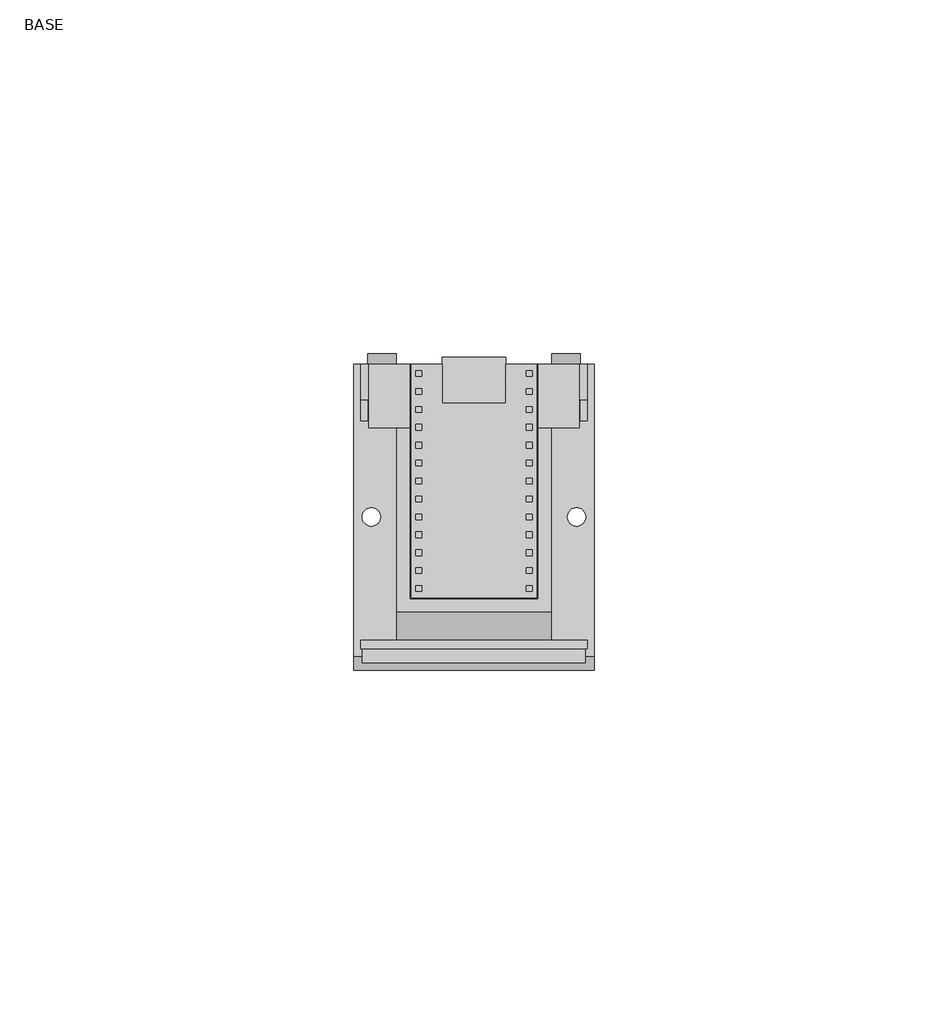
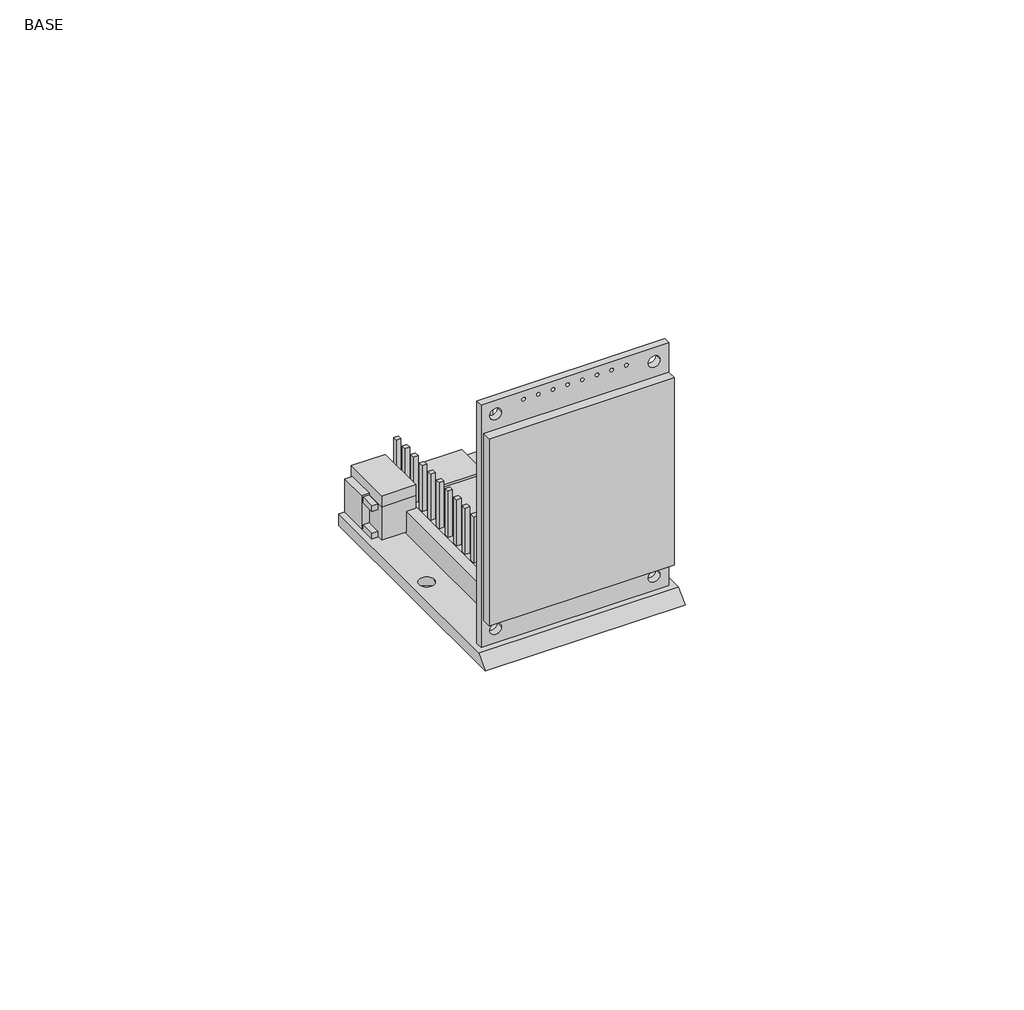
# One storey: 4 furniture elements, 1 proxy.
# Revit data of these elements (continued)
# Element 2 (IfcFurniture, "1.54TFT_SCREEN : 1.54TFT_SCREEN")
#   Phase Created = Fase 1
#   Materials on its faces: ".VIDRO"
# Element 3 (IfcFurniture, "PRO_MICRO-NRF52840 : PRO_MICRO-NRF52840")
#   Phase Created = Fase 1
#   Materials on its faces: ".CHIP"
# Elements 4, 5 (IfcFurniture, "PUSH_BUTTON_6x6 : PUSH_BUTTON_6x6")
#   Phase Created = Fase 1
#   Materials on its faces: ".BOTAO"
# Materials
#   "Areia": class "Genérico", colour RGB 191 183 178, transparency 0, Description = "Areia", Cost = 0
#   ".VIDRO": class "Vidro", colour RGB 165 190 164, transparency 0.4, Cost = 0
#   ".CHIP": class "Vidro", colour RGB 236 240 239, transparency 0.35, Cost = 0
#   ".BOTAO": class "Vidro", colour RGB 0 255 255, transparency 0.75, Cost = 0
